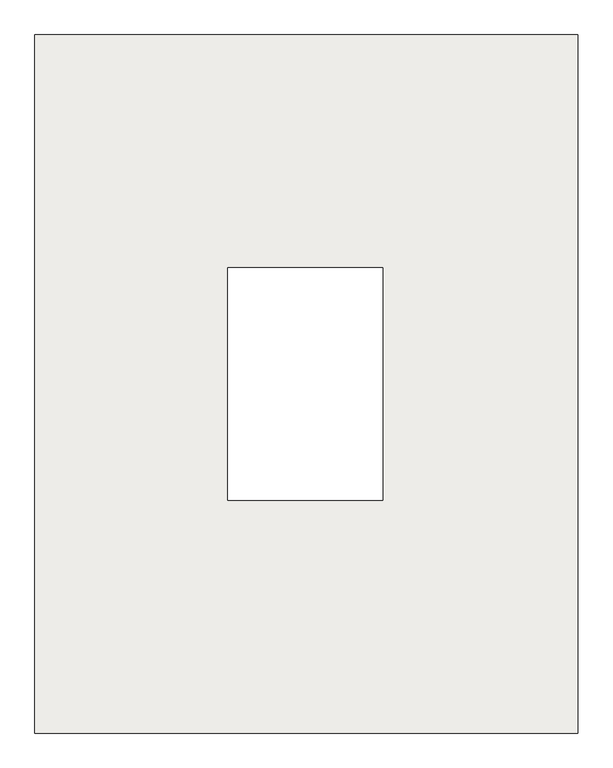
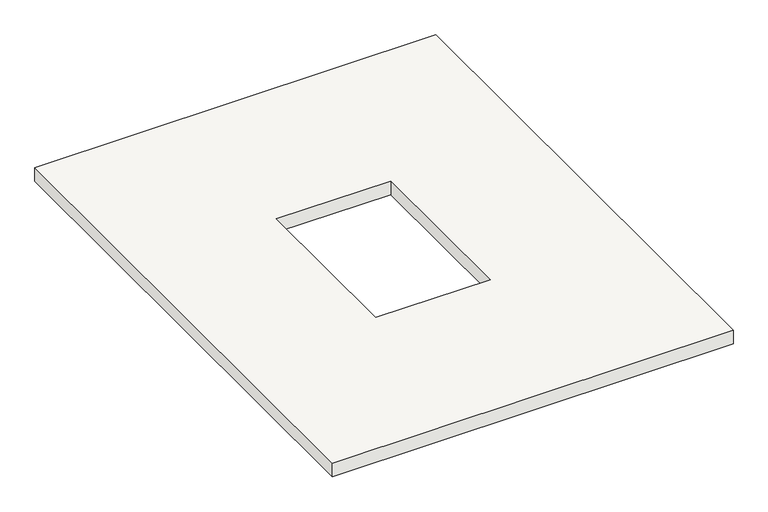
"""IFC4 building model written with IfcOpenShell, lengths in millimetres: slab geometry, Holzdecke : Holzdecke."""

from ifc_helpers import new_model, si_unit, frame, origin, place, context, project, spatial, polyline, outline, extrude, source, transform, mapped, element, save


def slab_87d51967(model_context):
    return source(origin(), model_context, "Body", "SweptSolid", [
        extrude(outline(polyline([(15500.0, 1547.1380981), (1500.0, 1547.1380981), (1500.0, 19550.0), (15500.0, 19550.0), (15500.0, 1547.1380981)]), holes=[polyline([(10475.0, 13550.0), (6475.0, 13550.0), (6475.0, 7550.0), (10475.0, 7550.0), (10475.0, 13550.0)])]), frame((0.0, 0.0, -500.0), z_axis=(0.0, 0.0, 1.0), x_axis=(1.0, 0.0, 0.0)), (0.0, 0.0, 1.0), 500.0),
    ])


if __name__ == "__main__":
    model = new_model("IFC4")
    model_context = context("Model", 3, world=origin())
    ifc_project = project(units=[si_unit("LENGTHUNIT", "METRE", prefix="MILLI")], contexts=[model_context])
    site = spatial("IfcSite", under=ifc_project)
    building = spatial("IfcBuilding", under=site)
    placement = place(None, origin())
    slab_shape = slab_87d51967(model_context)
    element("IfcSlab", 1, ObjectType="Holzdecke : Holzdecke", at=placement, inside=building, context=model_context, shape_type="MappedRepresentation", body=[
        mapped(slab_shape, transform((0.0, 0.0, 0.0), x_axis=(1.0, 0.0, 0.0), y_axis=(0.0, 1.0, 0.0), z_axis=(0.0, 0.0, 1.0))),
    ])
    save(model, "model.ifc")

# Revit data of these elements
# Type "Holzdecke : Holzdecke"
#   Abrechnungsart = "m²"
#   Allright_Bauteil_ID = "0110De 0783954323"
#   Bezeichnung = "Holzdecke"
#   Codetext = "D-HOLZBALKEN1\\"
#   Gewerk = "Zimmer- und Holzbauarbeiten"
#   Material = "Holz"
#   Objektname = "Brettstapeldecke"
#   NameOverride = "Holzdecke"
#   Reference = "Holzdecke"
#   Status = "NEW"
#   PitchAngle = 0.00°
#   ThermalTransmittance = 0.0000 BTU/(h·ft²·°F)
#   2D Interaktion = yes
#   Combustible = no
#   Compartmentation = no
#   IsExternal = no
#   LoadBearing = yes
# Element 1 (IfcSlab, "Holzdecke : Holzdecke")
#   Materials on its faces: "Default Floor"
# Materials
#   "Default Floor": class "Miscellaneous", colour RGB 128 128 128, transparency 0, Cost = 0
